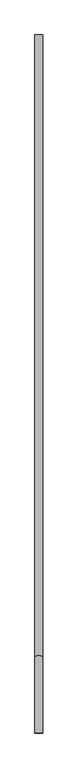
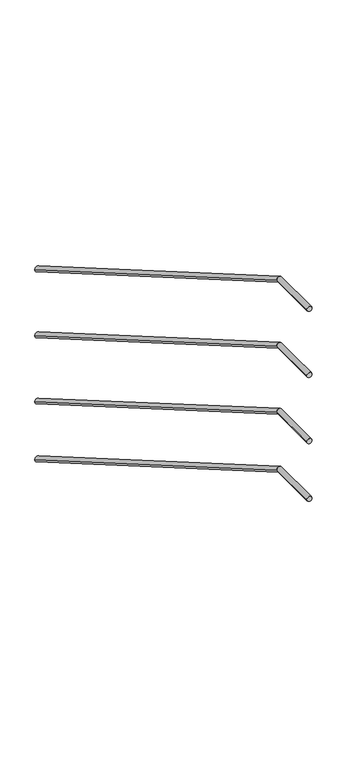
"""IFC4 building model written with IfcOpenShell, lengths in millimetres: railing geometry."""

from ifc_helpers import new_model, si_unit, frame, origin, place, context, project, spatial, circle_curve, ellipse_curve, source, transform, mapped, element, save
from ifc_brep_helpers import plane_surface, cylinder_surface, advanced_brep


def railing_95222ce5(model_context):
    return source(origin(), model_context, "Body", "AdvancedBrep", [
        advanced_brep(
        [(-340.4, 15799.5208589, 2729.6773196), (-310.4, 15799.5208589, 2729.6773196), (-340.4, 13395.4833005, 4124.9618634), (-310.4, 13395.4833005, 4124.9618634), (-340.4, 13099.5208589, 4124.9618634), (-310.4, 13099.5208589, 4124.9618634)],
        [
            (0, 1, ellipse_curve(frame((-325.4, 15799.5208589, 2729.6773196), z_axis=(0.0, 1.0, 0.0), x_axis=(0.0, 0.0, -1.0)), 17.3433672, 15.0)),
            (1, 0, ellipse_curve(frame((-325.4, 15799.5208589, 2729.6773196), z_axis=(0.0, 1.0, 0.0), x_axis=(0.0, 0.0, -1.0)), 17.3433672, 15.0)),
            (0, 2),
            (2, 3, ellipse_curve(frame((-325.4, 13395.4833005, 4124.9618634), z_axis=(0.0, 0.9656303515230847, -0.2599192648062161), x_axis=(0.0, -0.2599192648062165, -0.9656303515230846)), 15.5338945, 15.0)),
            (3, 1),
            (3, 2, ellipse_curve(frame((-325.4, 13395.4833005, 4124.9618634), z_axis=(0.0, 0.9656303515230847, -0.2599192648062161), x_axis=(0.0, -0.2599192648062165, -0.9656303515230846)), 15.5338945, 15.0)),
            (4, 5, circle_curve(frame((-325.4, 13099.5208589, 4124.9618634), z_axis=(0.0, -1.0, 0.0), x_axis=(1.0, 0.0, 0.0)), 15.0)),
            (5, 4, circle_curve(frame((-325.4, 13099.5208589, 4124.9618634), z_axis=(0.0, -1.0, 0.0), x_axis=(1.0, 0.0, 0.0)), 15.0)),
            (2, 4),
            (5, 3),
        ],
        [
            plane_surface(frame((-325.4, 15799.5208589, 2747.0206869), z_axis=(0.0, 1.0, 0.0), x_axis=(0.0, 0.0, -1.0))),
            cylinder_surface(frame((-325.4, 15791.991281, 2734.0474276), z_axis=(0.0, 0.8648839515651924, -0.5019718620848963), x_axis=(1.0, 0.0, 0.0)), 15.0),
            plane_surface(frame((-325.4, 13099.5208589, 4139.9618634), z_axis=(0.0, -1.0, 0.0), x_axis=(0.0, 0.0, -1.0))),
            cylinder_surface(frame((-325.4, 13399.5208589, 4124.9618634), z_axis=(0.0, 1.0, 0.0), x_axis=(1.0, 0.0, 0.0)), 15.0),
        ],
        [
            (0, [[1, 2]]),
            (1, [[-1, 3, 4, 5]]),
            (1, [[-2, -5, 6, -3]]),
            (2, [[7, 8]]),
            (3, [[-4, 9, -8, 10]]),
            (3, [[-6, -10, -7, -9]]),
        ],
    ),
        advanced_brep(
        [(-340.4, 15799.5208589, 1929.6773196), (-310.4, 15799.5208589, 1929.6773196), (-340.4, 13395.4833005, 3324.9618634), (-310.4, 13395.4833005, 3324.9618634), (-340.4, 13099.5208589, 3324.9618634), (-310.4, 13099.5208589, 3324.9618634)],
        [
            (0, 1, ellipse_curve(frame((-325.4, 15799.5208589, 1929.6773196), z_axis=(0.0, 1.0, 0.0), x_axis=(0.0, 0.0, -1.0)), 17.3433672, 15.0)),
            (1, 0, ellipse_curve(frame((-325.4, 15799.5208589, 1929.6773196), z_axis=(0.0, 1.0, 0.0), x_axis=(0.0, 0.0, -1.0)), 17.3433672, 15.0)),
            (0, 2),
            (2, 3, ellipse_curve(frame((-325.4, 13395.4833005, 3324.9618634), z_axis=(0.0, 0.9656303515230847, -0.2599192648062161), x_axis=(0.0, -0.2599192648062165, -0.9656303515230846)), 15.5338945, 15.0)),
            (3, 1),
            (3, 2, ellipse_curve(frame((-325.4, 13395.4833005, 3324.9618634), z_axis=(0.0, 0.9656303515230847, -0.2599192648062161), x_axis=(0.0, -0.2599192648062165, -0.9656303515230846)), 15.5338945, 15.0)),
            (4, 5, circle_curve(frame((-325.4, 13099.5208589, 3324.9618634), z_axis=(0.0, -1.0, 0.0), x_axis=(1.0, 0.0, 0.0)), 15.0)),
            (5, 4, circle_curve(frame((-325.4, 13099.5208589, 3324.9618634), z_axis=(0.0, -1.0, 0.0), x_axis=(1.0, 0.0, 0.0)), 15.0)),
            (2, 4),
            (5, 3),
        ],
        [
            plane_surface(frame((-325.4, 15799.5208589, 1947.0206869), z_axis=(0.0, 1.0, 0.0), x_axis=(0.0, 0.0, -1.0))),
            cylinder_surface(frame((-325.4, 15791.991281, 1934.0474276), z_axis=(0.0, 0.8648839515651924, -0.5019718620848963), x_axis=(1.0, 0.0, 0.0)), 15.0),
            plane_surface(frame((-325.4, 13099.5208589, 3339.9618634), z_axis=(0.0, -1.0, 0.0), x_axis=(0.0, 0.0, -1.0))),
            cylinder_surface(frame((-325.4, 13399.5208589, 3324.9618634), z_axis=(0.0, 1.0, 0.0), x_axis=(1.0, 0.0, 0.0)), 15.0),
        ],
        [
            (0, [[1, 2]]),
            (1, [[-1, 3, 4, 5]]),
            (1, [[-2, -5, 6, -3]]),
            (2, [[7, 8]]),
            (3, [[-4, 9, -8, 10]]),
            (3, [[-6, -10, -7, -9]]),
        ],
    ),
        advanced_brep(
        [(-340.4, 15799.5208589, 2329.6773196), (-310.4, 15799.5208589, 2329.6773196), (-340.4, 13395.4833005, 3724.9618634), (-310.4, 13395.4833005, 3724.9618634), (-340.4, 13099.5208589, 3724.9618634), (-310.4, 13099.5208589, 3724.9618634)],
        [
            (0, 1, ellipse_curve(frame((-325.4, 15799.5208589, 2329.6773196), z_axis=(0.0, 1.0, 0.0), x_axis=(0.0, 0.0, -1.0)), 17.3433672, 15.0)),
            (1, 0, ellipse_curve(frame((-325.4, 15799.5208589, 2329.6773196), z_axis=(0.0, 1.0, 0.0), x_axis=(0.0, 0.0, -1.0)), 17.3433672, 15.0)),
            (0, 2),
            (2, 3, ellipse_curve(frame((-325.4, 13395.4833005, 3724.9618634), z_axis=(0.0, 0.9656303515230847, -0.2599192648062161), x_axis=(0.0, -0.2599192648062165, -0.9656303515230846)), 15.5338945, 15.0)),
            (3, 1),
            (3, 2, ellipse_curve(frame((-325.4, 13395.4833005, 3724.9618634), z_axis=(0.0, 0.9656303515230847, -0.2599192648062161), x_axis=(0.0, -0.2599192648062165, -0.9656303515230846)), 15.5338945, 15.0)),
            (4, 5, circle_curve(frame((-325.4, 13099.5208589, 3724.9618634), z_axis=(0.0, -1.0, 0.0), x_axis=(1.0, 0.0, 0.0)), 15.0)),
            (5, 4, circle_curve(frame((-325.4, 13099.5208589, 3724.9618634), z_axis=(0.0, -1.0, 0.0), x_axis=(1.0, 0.0, 0.0)), 15.0)),
            (2, 4),
            (5, 3),
        ],
        [
            plane_surface(frame((-325.4, 15799.5208589, 2347.0206869), z_axis=(0.0, 1.0, 0.0), x_axis=(0.0, 0.0, -1.0))),
            cylinder_surface(frame((-325.4, 15791.991281, 2334.0474276), z_axis=(0.0, 0.8648839515651924, -0.5019718620848963), x_axis=(1.0, 0.0, 0.0)), 15.0),
            plane_surface(frame((-325.4, 13099.5208589, 3739.9618634), z_axis=(0.0, -1.0, 0.0), x_axis=(0.0, 0.0, -1.0))),
            cylinder_surface(frame((-325.4, 13399.5208589, 3724.9618634), z_axis=(0.0, 1.0, 0.0), x_axis=(1.0, 0.0, 0.0)), 15.0),
        ],
        [
            (0, [[1, 2]]),
            (1, [[-1, 3, 4, 5]]),
            (1, [[-2, -5, 6, -3]]),
            (2, [[7, 8]]),
            (3, [[-4, 9, -8, 10]]),
            (3, [[-6, -10, -7, -9]]),
        ],
    ),
        advanced_brep(
        [(-340.4, 15799.5208589, 1579.6773196), (-310.4, 15799.5208589, 1579.6773196), (-340.4, 13395.4833005, 2974.9618634), (-310.4, 13395.4833005, 2974.9618634), (-340.4, 13099.5208589, 2974.9618634), (-310.4, 13099.5208589, 2974.9618634)],
        [
            (0, 1, ellipse_curve(frame((-325.4, 15799.5208589, 1579.6773196), z_axis=(0.0, 1.0, 0.0), x_axis=(0.0, 0.0, -1.0)), 17.3433672, 15.0)),
            (1, 0, ellipse_curve(frame((-325.4, 15799.5208589, 1579.6773196), z_axis=(0.0, 1.0, 0.0), x_axis=(0.0, 0.0, -1.0)), 17.3433672, 15.0)),
            (0, 2),
            (2, 3, ellipse_curve(frame((-325.4, 13395.4833005, 2974.9618634), z_axis=(0.0, 0.9656303515230847, -0.2599192648062161), x_axis=(0.0, -0.2599192648062165, -0.9656303515230846)), 15.5338945, 15.0)),
            (3, 1),
            (3, 2, ellipse_curve(frame((-325.4, 13395.4833005, 2974.9618634), z_axis=(0.0, 0.9656303515230847, -0.2599192648062161), x_axis=(0.0, -0.2599192648062165, -0.9656303515230846)), 15.5338945, 15.0)),
            (4, 5, circle_curve(frame((-325.4, 13099.5208589, 2974.9618634), z_axis=(0.0, -1.0, 0.0), x_axis=(1.0, 0.0, 0.0)), 15.0)),
            (5, 4, circle_curve(frame((-325.4, 13099.5208589, 2974.9618634), z_axis=(0.0, -1.0, 0.0), x_axis=(1.0, 0.0, 0.0)), 15.0)),
            (2, 4),
            (5, 3),
        ],
        [
            plane_surface(frame((-325.4, 15799.5208589, 1597.0206869), z_axis=(0.0, 1.0, 0.0), x_axis=(0.0, 0.0, -1.0))),
            cylinder_surface(frame((-325.4, 15791.991281, 1584.0474276), z_axis=(0.0, 0.8648839515651924, -0.5019718620848963), x_axis=(1.0, 0.0, 0.0)), 15.0),
            plane_surface(frame((-325.4, 13099.5208589, 2989.9618634), z_axis=(0.0, -1.0, 0.0), x_axis=(0.0, 0.0, -1.0))),
            cylinder_surface(frame((-325.4, 13399.5208589, 2974.9618634), z_axis=(0.0, 1.0, 0.0), x_axis=(1.0, 0.0, 0.0)), 15.0),
        ],
        [
            (0, [[1, 2]]),
            (1, [[-1, 3, 4, 5]]),
            (1, [[-2, -5, 6, -3]]),
            (2, [[7, 8]]),
            (3, [[-4, 9, -8, 10]]),
            (3, [[-6, -10, -7, -9]]),
        ],
    ),
    ])


if __name__ == "__main__":
    model = new_model("IFC4")
    model_context = context("Model", 3, world=origin())
    ifc_project = project(units=[si_unit("LENGTHUNIT", "METRE", prefix="MILLI")], contexts=[model_context])
    site = spatial("IfcSite", under=ifc_project)
    building = spatial("IfcBuilding", under=site)
    placement = place(None, origin())
    railing_shape = railing_95222ce5(model_context)
    element("IfcRailing", 1, at=placement, inside=building, context=model_context, shape_type="MappedRepresentation", body=[
        mapped(railing_shape, transform((0.0, 0.0, 0.0), x_axis=(1.0, 0.0, 0.0), y_axis=(0.0, 1.0, 0.0), z_axis=(0.0, 0.0, 1.0))),
    ])
    save(model, "model.ifc")
